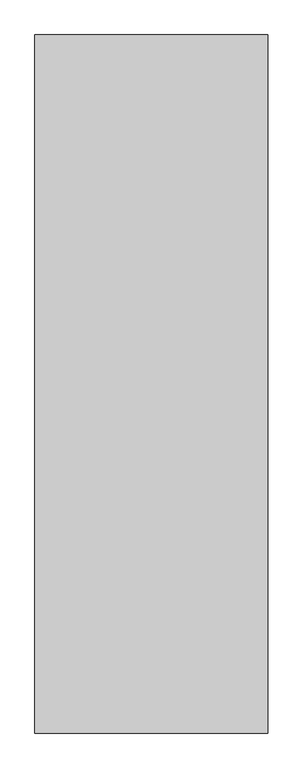
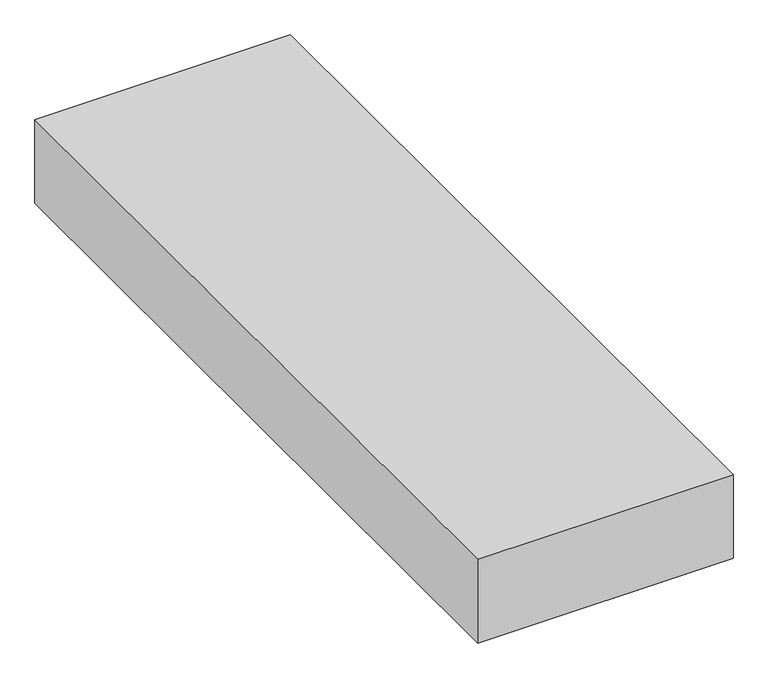
"""IFC4 building model written with IfcOpenShell, lengths in millimetres: proxy geometry, Space Planning Box_hec : Space Planning Box_hec."""

from ifc_helpers import new_model, si_unit, origin, origin_with_axes, place, context, project, spatial, polyline, outline, extrude, source, transform, mapped, element, save


def generic_models_083cc7c1(model_context):
    return source(origin(), model_context, "Body", "SweptSolid", [
        extrude(outline(polyline([(7500.0, 22500.0), (7500.0, -22500.0), (-7500.0, -22500.0), (-7500.0, 22500.0), (7500.0, 22500.0)])), origin_with_axes(), (0.0, 0.0, 1.0), 5200.0),
    ])


if __name__ == "__main__":
    model = new_model("IFC4")
    model_context = context("Model", 3, world=origin())
    ifc_project = project(units=[si_unit("LENGTHUNIT", "METRE", prefix="MILLI")], contexts=[model_context])
    site = spatial("IfcSite", under=ifc_project)
    building = spatial("IfcBuilding", under=site)
    placement = place(None, origin())
    generic_models_shape = generic_models_083cc7c1(model_context)
    element("IfcBuildingElementProxy", 1, Name="Space Planning Box_hec : Space Planning Box_hec", ObjectType="Space Planning Box_hec : Space Planning Box_hec", at=placement, inside=building, context=model_context, shape_type="MappedRepresentation", body=[
        mapped(generic_models_shape, transform((0.0, 0.0, 0.0), x_axis=(1.0, 0.0, 0.0), y_axis=(0.0, 1.0, 0.0), z_axis=(0.0, 0.0, 1.0))),
    ])
    save(model, "model.ifc")

# Revit data of these elements
# Type "Space Planning Box_hec : Space Planning Box_hec"
#   Type Comments = "..."
#   Room Name [instance default] = "?"
#   Interior Finish [instance default] = ""
#   Exterior Finish [instance default] = ""
#   Department [instance default] = ""
#   Assembly Code = "..."
#   ceiling height [instance default] = 0
#   Width [instance default] = 1524 mm
#   Program Area [instance default] = 0.00 m²
#   Length [instance default] = 1524 mm
#   Height [instance default] = 1524 mm
#   Area [instance default] = 2.32258 m²
#   Fill Color [instance default] = Cyan
#   Default Elevation = 0
# Element 1 (IfcBuildingElementProxy, "Space Planning Box_hec : Space Planning Box_hec")
#   Room Name = "Corridor"
#   Interior Finish = "IW1..N/A,,WB2..N/A,,FL6..N/A,,CL4..N/A"
#   Exterior Finish = "RF1..N/A,,EW1..N/A"
#   Department = "AR"
#   ceiling height = 2700
#   Width = 15000 mm
#   Program Area = 117.25 m²
#   Length = 45000 mm
#   Height = 5200 mm
#   Area = 675.00 m²
#   Materials on its faces: "Cyan"
# Materials
#   "Cyan": class "Generic", colour RGB 0 255 255, transparency 0.2, Cost = 0
